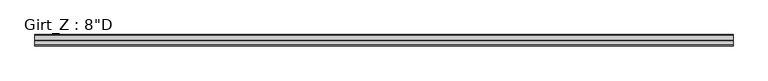
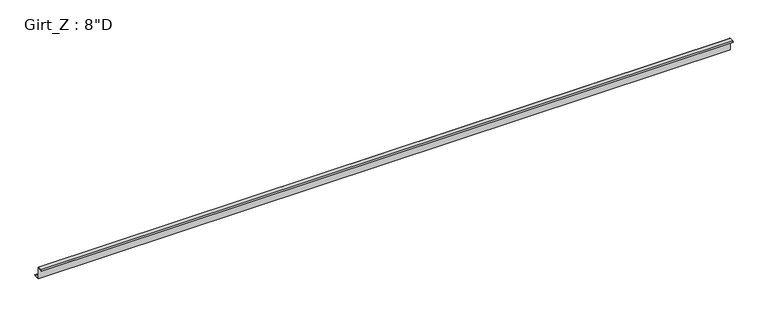
"""IFC4 building model written with IfcOpenShell, lengths in millimetres: beam geometry."""

import ifcopenshell
import ifcopenshell.guid

model = None  # the IFC model being written
_history = None  # IfcOwnerHistory: only IFC2X3 demands one
_inside = {}  # id of a spatial element -> (the spatial element, [elements in it])
_under = {}  # id of a project, library or spatial element -> (it, [spatial elements below it])
_declared = {}  # id of a project -> (the project, [libraries it declares])
_typed = {}  # id of a type object -> (the type object, [elements of that type])
_made_of = {}  # id of a material, layer set ... -> (it, [elements and type objects made of it])


def new_model(schema):
    """Start an empty IFC model of exactly this schema.

    Asked for "IFC4X3", IfcOpenShell would pick the latest addendum, in which some entities
    have other attributes; the version numbers below select the first issue.
    IFC2X3 requires an IfcOwnerHistory on every rooted entity: one is made here for all.
    """
    global model, _history
    if schema == "IFC4X3":
        model = ifcopenshell.file(schema_version=(4, 3, 0, 0))
    else:
        model = ifcopenshell.file(schema=schema)
    _inside.clear()
    _under.clear()
    _declared.clear()
    _typed.clear()
    _made_of.clear()
    _history = None
    if model.schema == "IFC2X3":
        org = make("IfcOrganization", Name="unknown")
        user = make(
            "IfcPersonAndOrganization",
            ThePerson=make("IfcPerson", FamilyName="unknown"),
            TheOrganization=org,
        )
        app = make(
            "IfcApplication",
            ApplicationDeveloper=org,
            Version="unknown",
            ApplicationFullName="unknown",
            ApplicationIdentifier="unknown",
        )
        _history = make(
            "IfcOwnerHistory",
            OwningUser=user,
            OwningApplication=app,
            ChangeAction="ADDED",
            CreationDate=0,
        )
    return model


def make(cls, **values):
    """One entity of the class cls with the attributes given. An attribute that is None is left unset."""
    return model.create_entity(
        cls, **{name: value for name, value in values.items() if value is not None}
    )


def rooted(cls, **values):
    """An entity with a GlobalId (a new one), such as an element, a storey or a relation."""
    return make(cls, GlobalId=ifcopenshell.guid.new(), OwnerHistory=_history, **values)


def si_unit(unit_type, name, prefix=None):
    """IfcSIUnit, for example si_unit("LENGTHUNIT", "METRE", prefix="MILLI")."""
    return make("IfcSIUnit", UnitType=unit_type, Prefix=prefix, Name=name)


def assignment(units):
    """IfcUnitAssignment: the units of a project."""
    return None if units is None else make("IfcUnitAssignment", Units=units)


def point(xyz):
    """IfcCartesianPoint."""
    return None if xyz is None else make("IfcCartesianPoint", Coordinates=xyz)


def direction(xyz):
    """IfcDirection."""
    return None if xyz is None else make("IfcDirection", DirectionRatios=xyz)


def frame(location, z_axis=None, x_axis=None):
    """IfcAxis2Placement3D, a coordinate frame: its origin and axes. An axis left out is left unset."""
    return make(
        "IfcAxis2Placement3D",
        Location=point(location),
        Axis=direction(z_axis),
        RefDirection=direction(x_axis),
    )


def frame_2d(location, x_axis=None):
    """IfcAxis2Placement2D, a coordinate frame in the plane: its origin and x axis."""
    return make(
        "IfcAxis2Placement2D", Location=point(location), RefDirection=direction(x_axis)
    )


def origin():
    """The frame at (0, 0, 0) with its axes left unset."""
    return frame((0.0, 0.0, 0.0))


def place(relative_to, where):
    """IfcLocalPlacement: puts the frame where relative to a parent placement (None: the world)."""
    return make(
        "IfcLocalPlacement", PlacementRelTo=relative_to, RelativePlacement=where
    )


def context(
    kind, dimensions, precision=None, world=None, true_north=None, identifier=None
):
    """IfcGeometricRepresentationContext, for example the 3D "Model" context."""
    return make(
        "IfcGeometricRepresentationContext",
        ContextIdentifier=identifier,
        ContextType=kind,
        CoordinateSpaceDimension=dimensions,
        Precision=precision,
        WorldCoordinateSystem=world,
        TrueNorth=true_north,
    )


def project(units=None, contexts=None):
    """IfcProject with its units and contexts."""
    return rooted(
        "IfcProject",
        Name="project",
        RepresentationContexts=contexts,
        UnitsInContext=assignment(units),
    )


def spatial(cls, under=None, at=None, **own):
    """A site, building, storey or space (cls), placed at a placement, below another one or the project."""
    s = rooted(cls, ObjectPlacement=at, **own)
    if under is not None:
        _under.setdefault(under.id(), (under, []))[1].append(s)
    return s


def polyline(points):
    """IfcPolyline through the points."""
    return make("IfcPolyline", Points=[point(p) for p in points])


def circle_curve(where, radius):
    """IfcCircle in the frame where."""
    return make("IfcCircle", Position=where, Radius=radius)


def trimmed(basis, trim1, trim2, sense, master):
    """IfcTrimmedCurve: the piece of a basis curve between two trims."""
    return make(
        "IfcTrimmedCurve",
        BasisCurve=basis,
        Trim1=trim1,
        Trim2=trim2,
        SenseAgreement=sense,
        MasterRepresentation=master,
    )


def segment(curve, same_sense, transition):
    """IfcCompositeCurveSegment."""
    return make(
        "IfcCompositeCurveSegment",
        Transition=transition,
        SameSense=same_sense,
        ParentCurve=curve,
    )


def composite_curve(segments, self_intersect=None):
    """IfcCompositeCurve: segments joined end to end."""
    return make("IfcCompositeCurve", Segments=segments, SelfIntersect=self_intersect)


def outline(outer, holes=None, kind="AREA"):
    """IfcArbitraryClosedProfileDef: a profile drawn as a closed curve; with holes, ...WithVoids."""
    if holes is None:
        return make("IfcArbitraryClosedProfileDef", ProfileType=kind, OuterCurve=outer)
    return make(
        "IfcArbitraryProfileDefWithVoids",
        ProfileType=kind,
        OuterCurve=outer,
        InnerCurves=holes,
    )


def extrude(swept, where, along, depth):
    """IfcExtrudedAreaSolid: the profile swept, set in the frame where, extruded along a direction by depth."""
    return make(
        "IfcExtrudedAreaSolid",
        SweptArea=swept,
        Position=where,
        ExtrudedDirection=direction(along),
        Depth=depth,
    )


def shape(context_of_items, identifier, shape_type, items):
    """IfcShapeRepresentation: the items that make up one representation, for example the "Body"."""
    return make(
        "IfcShapeRepresentation",
        ContextOfItems=context_of_items,
        RepresentationIdentifier=identifier,
        RepresentationType=shape_type,
        Items=items,
    )


def source(mapping_origin, context_of_items, identifier, shape_type, items):
    """IfcRepresentationMap: a shape defined once, which mapped items show again and again."""
    return make(
        "IfcRepresentationMap",
        MappingOrigin=mapping_origin,
        MappedRepresentation=shape(context_of_items, identifier, shape_type, items),
    )


def transform(
    local_origin,
    x_axis=None,
    y_axis=None,
    z_axis=None,
    scale=None,
    scale2=None,
    scale3=None,
    uniform=True,
):
    """IfcCartesianTransformationOperator3D, or its non-uniform kind. x_axis, y_axis, z_axis: its Axis1, 2, 3."""
    if uniform:
        return make(
            "IfcCartesianTransformationOperator3D",
            Axis1=direction(x_axis),
            Axis2=direction(y_axis),
            LocalOrigin=point(local_origin),
            Scale=scale,
            Axis3=direction(z_axis),
        )
    return make(
        "IfcCartesianTransformationOperator3DnonUniform",
        Axis1=direction(x_axis),
        Axis2=direction(y_axis),
        LocalOrigin=point(local_origin),
        Scale=scale,
        Axis3=direction(z_axis),
        Scale2=scale2,
        Scale3=scale3,
    )


def mapped(mapping_source, mapping_target):
    """IfcMappedItem: shows the shape of a source again, moved by a transform."""
    return make(
        "IfcMappedItem", MappingSource=mapping_source, MappingTarget=mapping_target
    )


def made_of(thing, what):
    """Note that an element or type object is made of a material, layer set ...; save() writes the relation."""
    if what is not None:
        _made_of.setdefault(what.id(), (what, []))[1].append(thing)
    return thing


def element(
    cls,
    number,
    at=None,
    inside=None,
    cuts=None,
    type_object=None,
    material=None,
    context=None,
    identifier="Body",
    shape_type=None,
    held_by="IfcProductDefinitionShape",
    body=None,
    shapes=None,
    **own,
):
    """One element of the class cls, such as IfcWall. Its Tag is "e" and its number.

    at: its placement. inside: the storey or other place that contains it. cuts: it is an
    opening in that element (IfcRelVoidsElement). A single representation is given by context,
    identifier, shape_type and body (its items); several are given by shapes. held_by: the class
    of the entity that holds the representations. save() writes the other relations.
    """
    e = rooted(cls, Tag="e%d" % number, ObjectPlacement=at, **own)
    if body is not None:
        shapes = [shape(context, identifier, shape_type, body)]
    if shapes is not None:
        e.Representation = make(held_by, Representations=shapes)
    if inside is not None:
        _inside.setdefault(inside.id(), (inside, []))[1].append(e)
    if cuts is not None:
        rooted(
            "IfcRelVoidsElement", RelatingBuildingElement=cuts, RelatedOpeningElement=e
        )
    if type_object is not None:
        _typed.setdefault(type_object.id(), (type_object, []))[1].append(e)
    return made_of(e, material)


def aggregate(whole, parts):
    """IfcRelAggregates: a whole, such as a stair, and the parts it consists of."""
    return rooted("IfcRelAggregates", RelatingObject=whole, RelatedObjects=parts)


def save(model, path):
    """Write the relations noted so far, then the file.

    IfcRelAggregates (storeys below a building ...), IfcRelContainedInSpatialStructure (elements
    in a storey), IfcRelDefinesByType, IfcRelAssociatesMaterial and IfcRelDeclares: one each for
    every whole, place, type object, material and project.
    """
    for whole, parts in _under.values():
        aggregate(whole, parts)
    for where, things in _inside.values():
        rooted(
            "IfcRelContainedInSpatialStructure",
            RelatedElements=things,
            RelatingStructure=where,
        )
    for kind, things in _typed.values():
        rooted("IfcRelDefinesByType", RelatedObjects=things, RelatingType=kind)
    for what, things in _made_of.values():
        rooted("IfcRelAssociatesMaterial", RelatedObjects=things, RelatingMaterial=what)
    for by, libraries in _declared.values():
        rooted("IfcRelDeclares", RelatingContext=by, RelatedDefinitions=libraries)
    model.write(path)


def beam_65b613bf(model_context):
    return source(origin(), model_context, "Body", "SweptSolid", [
        extrude(outline(composite_curve([segment(polyline([(-77.9859375, 101.6), (-3.3734375, 101.6)]), True, "CONTINUOUS"), segment(trimmed(circle_curve(frame_2d((-3.3734375, 96.8375)), 4.7625), [point((-3.3734375, 101.6))], [point((1.3890625, 96.8375))], False, "CARTESIAN"), True, "CONTINUOUS"), segment(polyline([(1.3890625, 96.8375), (1.3890625, -96.8389339)]), True, "CONTINUOUS"), segment(trimmed(circle_curve(frame_2d((3.3748024, -96.8389339)), 1.9857399), [point((1.3890625, -96.8389339))], [point((3.2694106, -98.821875))], True, "CARTESIAN"), True, "CONTINUOUS"), segment(polyline([(3.2694106, -98.821875), (83.0404765, -98.821875), (94.4528742, -85.221109), (96.5810415, -87.0068534), (84.3359375, -101.6), (-1.3890625, -101.6), (-1.3890625, 96.8381931)]), True, "CONTINUOUS"), segment(trimmed(circle_curve(frame_2d((-3.3741066, 96.8381931)), 1.9850441), [point((-1.3890625, 96.8381931))], [point((-3.3005807, 98.821875))], True, "CARTESIAN"), True, "CONTINUOUS"), segment(polyline([(-3.3005807, 98.821875), (-76.6904765, 98.821875), (-88.1028742, 85.221109), (-90.2310415, 87.0068534), (-77.9859375, 101.6)]), True, "CONTINUOUS")], self_intersect=False)), frame((-5822.9499994, 0.0, 0.0), z_axis=(1.0, 0.0, 0.0), x_axis=(0.0, 1.0, 0.0)), (0.0, 0.0, 1.0), 11658.5999994),
    ])


if __name__ == "__main__":
    model = new_model("IFC4")
    model_context = context("Model", 3, world=origin())
    ifc_project = project(units=[si_unit("LENGTHUNIT", "METRE", prefix="MILLI")], contexts=[model_context])
    site = spatial("IfcSite", under=ifc_project)
    building = spatial("IfcBuilding", under=site)
    placement = place(None, origin())
    beam_shape = beam_65b613bf(model_context)
    element("IfcBeam", 1, ObjectType="Girt_Z : 8\"D", at=placement, inside=building, context=model_context, shape_type="MappedRepresentation", body=[
        mapped(beam_shape, transform((0.0, 0.0, 0.0), x_axis=(1.0, 0.0, 0.0), y_axis=(0.0, 1.0, 0.0), z_axis=(0.0, 0.0, 1.0))),
    ])
    save(model, "model.ifc")

# Revit data of these elements
# Type "Girt_Z : 8\"D"
#   half leg = 0' - 1 11/16"
#   Web_Thickness = 0' - 0 7/64"
#   Length [instance default] = 10' - 0"
#   Leg_2 = 0' - 3 3/8"
#   Leg_1 = 0' - 3 1/8"
#   Height = 0' - 8"
#   Structural Material [instance default] = none
